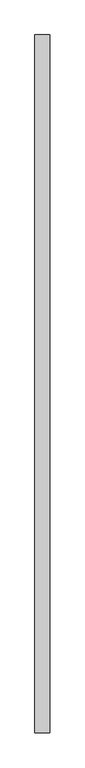
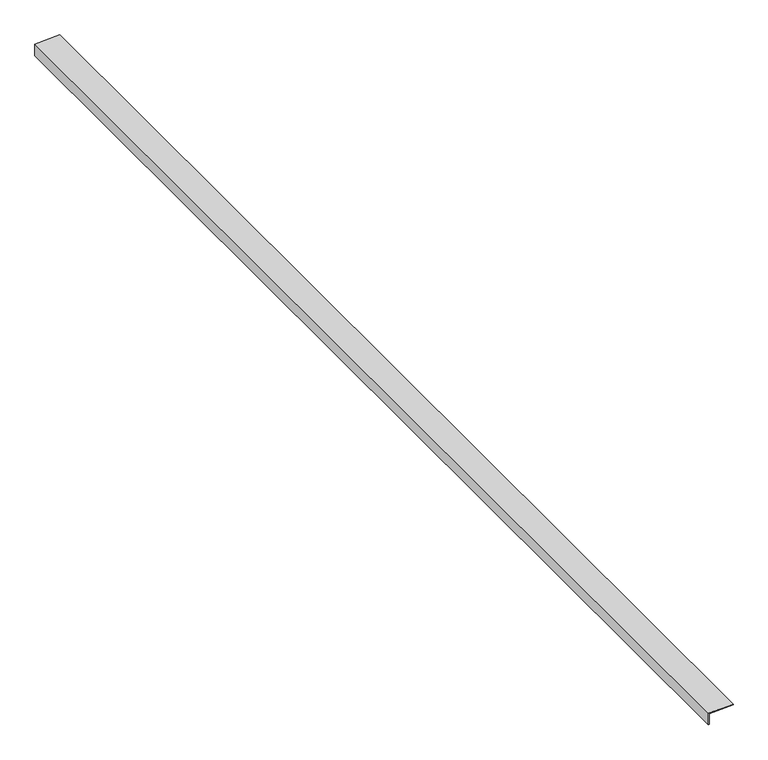
"""IFC4 building model written with IfcOpenShell, lengths in millimetres: proxy geometry, Generic Models 7:Generic Models 1:8:Generic Models 1:8 : Generic Models 7:Generic Models 1:337419:52 : Generic Models 7:Generic Models 1:8:Generic Models 1:8 : Generic Models 7:Generic Models 1:337419:315935."""

from ifc_helpers import new_model, si_unit, frame, origin, place, context, project, spatial, polyline, outline, extrude, source, transform, mapped, element, save


def generic_models_7e1a833f(model_context):
    return source(origin(), model_context, "Body", "SweptSolid", [
        extrude(outline(polyline([(3665.1571615, 560245.7438789), (3712.5900973, 560245.7438789), (3716.7350684, 560345.2231854), (3720.2423053, 560345.0770505), (3715.9571615, 560242.2335989), (3665.1571615, 560242.2335989), (3665.1571615, 560245.7438789)])), frame((0.0, -548060.3163841, 0.0), z_axis=(0.0, 1.0, 0.0), x_axis=(0.0, 0.0, 1.0)), (0.0, 0.0, 1.0), 4876.8),
    ])


if __name__ == "__main__":
    model = new_model("IFC4")
    model_context = context("Model", 3, world=origin())
    ifc_project = project(units=[si_unit("LENGTHUNIT", "METRE", prefix="MILLI")], contexts=[model_context])
    site = spatial("IfcSite", under=ifc_project)
    building = spatial("IfcBuilding", under=site)
    placement = place(None, origin())
    generic_models_shape = generic_models_7e1a833f(model_context)
    element("IfcBuildingElementProxy", 1, Name="Generic Models 7:Generic Models 1:8:Generic Models 1:8 : Generic Models 7:Generic Models 1:337419:52 : Generic Models 7:Generic Models 1:8:Generic Models 1:8 : Generic Models 7:Generic Models 1:337419:315935", ObjectType="Generic Models 7:Generic Models 1:8:Generic Models 1:8 : Generic Models 7:Generic Models 1:337419:52 : Generic Models 7:Generic Models 1:8:Generic Models 1:8 : Generic Models 7:Generic Models 1:337419:315935", at=placement, inside=building, context=model_context, shape_type="MappedRepresentation", body=[
        mapped(generic_models_shape, transform((0.0, 0.0, 0.0), x_axis=(1.0, 0.0, 0.0), y_axis=(0.0, 1.0, 0.0), z_axis=(0.0, 0.0, 1.0))),
    ])
    save(model, "model.ifc")

# Revit data of these elements
# Type "Generic Models 7:Generic Models 1:8:Generic Models 1:8 : Generic Models 7:Generic Models 1:337419:52 : Generic Models 7:Generic Models 1:8:Generic Models 1:8 : Generic Models 7:Generic Models 1:337419:315935"
#   NameOverride = "Generic Models 7:Generic Models 1:8:Generic Models 1:8 : Generic Models 7:Generic Models 1:337419:315935"
#   ObjectTypeOverride = "Generic Models 1:8 : Generic Models 7:Generic Models 1:337419"
#   Reference = "Generic Models 1"
#   Tag = "315935"
# Element 1 (IfcBuildingElementProxy, "Generic Models 7:Generic Models 1:8:Generic Models 1:8 : Generic Models 7:Generic Models 1:337419:52 : Generic Models 7:Generic Models 1:8:Generic Models 1:8 : Generic Models 7:Generic Models 1:337419:315935")
#   Materials on its faces: "11 GA. ALUM. BRAKE METAL (ALIGN WITH B.M. @ STOREFRONT/RESIN/POLYCARBONATE)"
# Materials
#   "11 GA. ALUM. BRAKE METAL (ALIGN WITH B.M. @ STOREFRONT/RESIN/POLYCARBONATE)": class "Unassigned", colour RGB 210 209 208, transparency 0, Cost = 0
